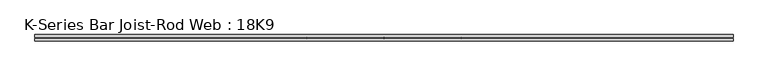
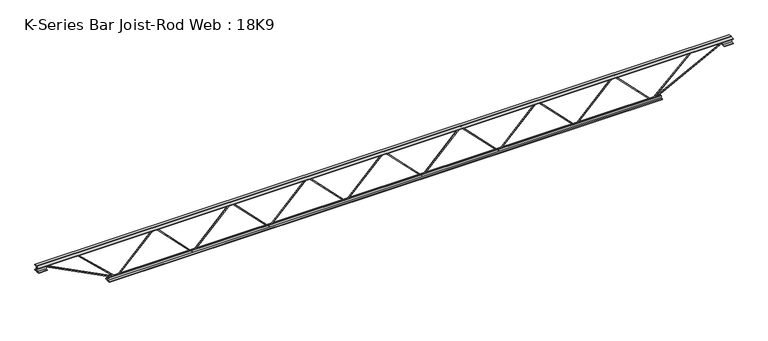
"""IFC4 building model written with IfcOpenShell, lengths in millimetres: beam geometry, K-Series Bar Joist-Rod Web : 18K9."""

from ifc_helpers import new_model, si_unit, frame, origin, place, context, project, spatial, polyline, outline, extrude, source, transform, mapped, element, save


def k_series_bar_joist_rod_web_18k9_9537e142(model_context):
    return source(origin(), model_context, "Body", "SweptSolid", [
        extrude(outline(polyline([(-217.4875, 1320.9133929), (-227.0125, 1320.9133929), (-227.0125, 1326.0946579), (217.4875, 1760.0491222), (217.4875, 1762.3865921), (-227.0125, 2196.3410564), (-227.0125, 2201.5223214), (-217.4875, 2201.5223214), (-217.4875, 2200.3535864), (227.0125, 1766.3991222), (227.0125, 1756.0365921), (-217.4875, 1322.0821278), (-217.4875, 1320.9133929)])), frame((0.0, -4.7625, 0.0), z_axis=(0.0, 1.0, 0.0), x_axis=(0.0, 0.0, 1.0)), (0.0, 0.0, 1.0), 9.525),
        extrude(outline(polyline([(-217.4875, 440.3044643), (-227.0125, 440.3044643), (-227.0125, 445.4857293), (217.4875, 879.4401936), (217.4875, 881.7776636), (-227.0125, 1315.7321278), (-227.0125, 1320.9133929), (-217.4875, 1320.9133929), (-217.4875, 1319.7446579), (227.0125, 885.7901936), (227.0125, 875.4276636), (-217.4875, 441.4731993), (-217.4875, 440.3044643)])), frame((0.0, -4.7625, 0.0), z_axis=(0.0, 1.0, 0.0), x_axis=(0.0, 0.0, 1.0)), (0.0, 0.0, 1.0), 9.525),
        extrude(outline(polyline([(-217.4875, -440.3044643), (-227.0125, -440.3044643), (-227.0125, -435.1231993), (217.4875, -1.168735), (217.4875, 1.168735), (-227.0125, 435.1231993), (-227.0125, 440.3044643), (-217.4875, 440.3044643), (-217.4875, 439.1357293), (227.0125, 5.181265), (227.0125, -5.181265), (-217.4875, -439.1357293), (-217.4875, -440.3044643)])), frame((0.0, -4.7625, 0.0), z_axis=(0.0, 1.0, 0.0), x_axis=(0.0, 0.0, 1.0)), (0.0, 0.0, 1.0), 9.525),
        extrude(outline(polyline([(-217.4875, -1320.9133929), (-227.0125, -1320.9133929), (-227.0125, -1315.7321278), (217.4875, -881.7776636), (217.4875, -879.4401936), (-227.0125, -445.4857293), (-227.0125, -440.3044643), (-217.4875, -440.3044643), (-217.4875, -441.4731993), (227.0125, -875.4276636), (227.0125, -885.7901936), (-217.4875, -1319.7446579), (-217.4875, -1320.9133929)])), frame((0.0, -4.7625, 0.0), z_axis=(0.0, 1.0, 0.0), x_axis=(0.0, 0.0, 1.0)), (0.0, 0.0, 1.0), 9.525),
        extrude(outline(polyline([(-217.4875, -2201.5223214), (-227.0125, -2201.5223214), (-227.0125, -2196.3410564), (217.4875, -1762.3865921), (217.4875, -1760.0491222), (-227.0125, -1326.0946579), (-227.0125, -1320.9133929), (-217.4875, -1320.9133929), (-217.4875, -1322.0821278), (227.0125, -1756.0365921), (227.0125, -1766.3991222), (-217.4875, -2200.3535864), (-217.4875, -2201.5223214)])), frame((0.0, -4.7625, 0.0), z_axis=(0.0, 1.0, 0.0), x_axis=(0.0, 0.0, 1.0)), (0.0, 0.0, 1.0), 9.525),
        extrude(outline(polyline([(-217.4875, 2201.5223214), (-227.0125, 2201.5223214), (-227.0125, 2206.7035864), (217.4875, 2640.6580507), (217.4875, 2642.9955207), (-227.0125, 3076.949985), (-227.0125, 3082.13125), (-217.4875, 3082.13125), (-217.4875, 3080.962515), (227.0125, 2647.0080507), (227.0125, 2636.6455207), (-217.4875, 2202.6910564), (-217.4875, 2201.5223214)])), frame((0.0, -4.7625, 0.0), z_axis=(0.0, 1.0, 0.0), x_axis=(0.0, 0.0, 1.0)), (0.0, 0.0, 1.0), 9.525),
        extrude(outline(polyline([(-217.4875, -3082.13125), (-227.0125, -3082.13125), (-227.0125, -3076.949985), (217.4875, -2642.9955207), (217.4875, -2640.6580507), (-227.0125, -2206.7035864), (-227.0125, -2201.5223214), (-217.4875, -2201.5223214), (-217.4875, -2202.6910564), (227.0125, -2636.6455207), (227.0125, -2647.0080507), (-217.4875, -3080.962515), (-217.4875, -3082.13125)])), frame((0.0, -4.7625, 0.0), z_axis=(0.0, 1.0, 0.0), x_axis=(0.0, 0.0, 1.0)), (0.0, 0.0, 1.0), 9.525),
        extrude(outline(polyline([(4.7625, 228.6), (36.5125, 228.6), (36.5125, 222.25), (11.1125, 222.25), (11.1125, 196.85), (4.7625, 196.85), (4.7625, 228.6)])), frame((-3996.53125, 0.0, 0.0), z_axis=(1.0, 0.0, 0.0), x_axis=(0.0, 1.0, 0.0)), (0.0, 0.0, 1.0), 7993.0625),
        extrude(outline(polyline([(-4.7625, 228.6), (-4.7625, 196.85), (-11.1125, 196.85), (-11.1125, 222.25), (-36.5125, 222.25), (-36.5125, 228.6), (-4.7625, 228.6)])), frame((-3996.53125, 0.0, 0.0), z_axis=(1.0, 0.0, 0.0), x_axis=(0.0, 1.0, 0.0)), (0.0, 0.0, 1.0), 7993.0625),
        extrude(outline(polyline([(-4.7625, 165.1), (-36.5125, 165.1), (-36.5125, 171.45), (-11.1125, 171.45), (-11.1125, 196.85), (-4.7625, 196.85), (-4.7625, 165.1)])), frame((-3996.53125, 0.0, 0.0), z_axis=(1.0, 0.0, 0.0), x_axis=(0.0, 1.0, 0.0)), (0.0, 0.0, 1.0), 101.6),
        extrude(outline(polyline([(36.5125, 165.1), (4.7625, 165.1), (4.7625, 196.85), (11.1125, 196.85), (11.1125, 171.45), (36.5125, 171.45), (36.5125, 165.1)])), frame((-3996.53125, 0.0, 0.0), z_axis=(1.0, 0.0, 0.0), x_axis=(0.0, 1.0, 0.0)), (0.0, 0.0, 1.0), 101.6),
        extrude(outline(polyline([(4.7625, 165.1), (4.7625, 196.85), (11.1125, 196.85), (11.1125, 171.45), (36.5125, 171.45), (36.5125, 165.1), (4.7625, 165.1)])), frame((3894.93125, 0.0, 0.0), z_axis=(1.0, 0.0, 0.0), x_axis=(0.0, 1.0, 0.0)), (0.0, 0.0, 1.0), 101.6),
        extrude(outline(polyline([(-4.7625, 165.1), (-36.5125, 165.1), (-36.5125, 171.45), (-11.1125, 171.45), (-11.1125, 196.85), (-4.7625, 196.85), (-4.7625, 165.1)])), frame((3894.93125, 0.0, 0.0), z_axis=(1.0, 0.0, 0.0), x_axis=(0.0, 1.0, 0.0)), (0.0, 0.0, 1.0), 101.6),
        extrude(outline(polyline([(4.7625, -228.6), (4.7625, -196.85), (11.1125, -196.85), (11.1125, -222.25), (36.5125, -222.25), (36.5125, -228.6), (4.7625, -228.6)])), frame((-3183.73125, 0.0, 0.0), z_axis=(1.0, 0.0, 0.0), x_axis=(0.0, 1.0, 0.0)), (0.0, 0.0, 1.0), 6367.4625),
        extrude(outline(polyline([(-4.7625, -228.6), (-36.5125, -228.6), (-36.5125, -222.25), (-11.1125, -222.25), (-11.1125, -196.85), (-4.7625, -196.85), (-4.7625, -228.6)])), frame((-3183.73125, 0.0, 0.0), z_axis=(1.0, 0.0, 0.0), x_axis=(0.0, 1.0, 0.0)), (0.0, 0.0, 1.0), 6367.4625),
        extrude(outline(polyline([(0.0, -9.525), (0.0, 0.0), (914.4881902, 0.0), (914.4881902, -9.525), (0.0, -9.525)])), frame((-3897.113852, 4.7625, 192.6170749), z_axis=(0.45828913319472697, 0.0, 0.8888031674086371), x_axis=(0.8888031674086371, 0.0, -0.45828913319472697)), (0.0, 0.0, 1.0), 9.525),
        extrude(outline(polyline([(0.0, -9.525), (0.0, 0.0), (607.8756708, 0.0), (607.8756708, -9.525), (0.0, -9.525)])), frame((-3525.7192208, 4.7625, 193.4003636), z_axis=(0.689450195268687, 0.0, 0.724333092053628), x_axis=(0.724333092053628, 0.0, -0.689450195268687)), (0.0, 0.0, 1.0), 9.525),
        extrude(outline(polyline([(0.0, -9.525), (0.0, 0.0), (914.4881902, 0.0), (914.4881902, -9.525), (0.0, -9.525)])), frame((3897.113852, -4.7625, 192.6170749), z_axis=(-0.45828913319471637, 0.0, 0.8888031674086426), x_axis=(-0.8888031674086426, 0.0, -0.45828913319471637)), (0.0, 0.0, 1.0), 9.525),
        extrude(outline(polyline([(0.0, -9.525), (0.0, 0.0), (607.8756708, 0.0), (607.8756708, -9.525), (0.0, -9.525)])), frame((3525.7192208, -4.7625, 193.4003636), z_axis=(-0.6894501952686827, 0.0, 0.724333092053632), x_axis=(-0.724333092053632, 0.0, -0.6894501952686827)), (0.0, 0.0, 1.0), 9.525),
    ])


if __name__ == "__main__":
    model = new_model("IFC4")
    model_context = context("Model", 3, world=origin())
    ifc_project = project(units=[si_unit("LENGTHUNIT", "METRE", prefix="MILLI")], contexts=[model_context])
    site = spatial("IfcSite", under=ifc_project)
    building = spatial("IfcBuilding", under=site)
    placement = place(None, origin())
    k_series_bar_joist_rod_web_18k9_shape = k_series_bar_joist_rod_web_18k9_9537e142(model_context)
    element("IfcBeam", 1, ObjectType="K-Series Bar Joist-Rod Web : 18K9", at=placement, inside=building, context=model_context, shape_type="MappedRepresentation", body=[
        mapped(k_series_bar_joist_rod_web_18k9_shape, transform((0.0, 0.0, 0.0), x_axis=(1.0, 0.0, 0.0), y_axis=(0.0, 1.0, 0.0), z_axis=(0.0, 0.0, 1.0))),
    ])
    save(model, "model.ifc")

# Revit data of these elements
# Type "K-Series Bar Joist-Rod Web : 18K9"
#   Assembly Code = "B1010350"
#   Wt = 10.2
#   Web Thickness = 0' - 0 3/8"
#   Start Offset [instance default] = 0' - 0"
#   Start Extension [instance default] = 0' - 0"
#   Seat Length = 0' - 4"
#   Seat Depth = 0' - 2 1/2"
#   PanelArrayLength [instance default] = 18' - 0"
#   Panel [instance default] = 3' - 0"
#   End Offset [instance default] = 0' - 0"
#   End Extension [instance default] = 0' - 0"
#   End Panel = 3' - 0"
#   Cord Leg = 0' - 1 1/4"
#   Chord Thickness = 0' - 0 1/4"
#   Length [instance default] = 24' - 0"
#   Depth = 1' - 6"
#   PanelArrayNum [instance default] = 6
#   Structural Material = none
# Element 1 (IfcBeam, "K-Series Bar Joist-Rod Web : 18K9")
#   PanelArrayLength = 20' - 2 11/16"
#   Panel = 2' - 10.66964"
#   PanelArrayNum = 7
